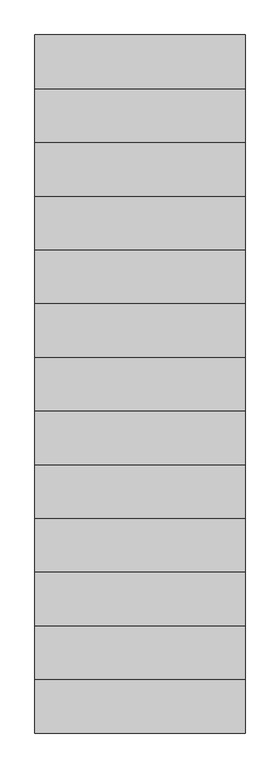
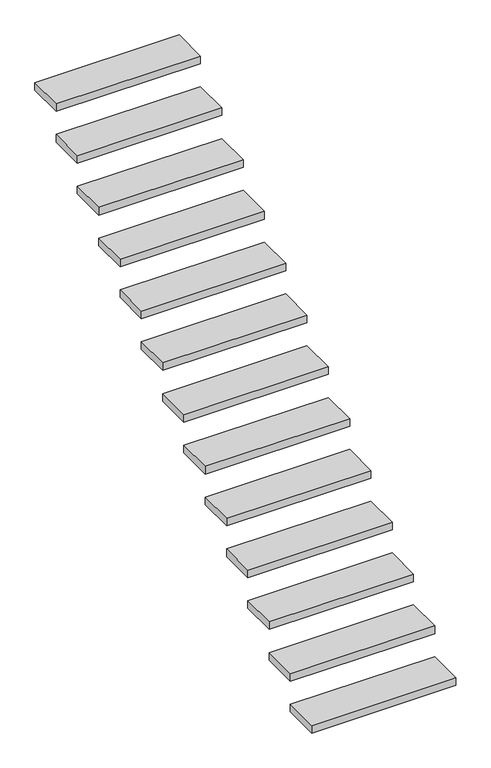
"""IFC4 building model written with IfcOpenShell, lengths in millimetres: stair geometry,   150832 :   150832."""

import ifcopenshell
import ifcopenshell.guid

model = None  # the IFC model being written
_history = None  # IfcOwnerHistory: only IFC2X3 demands one
_inside = {}  # id of a spatial element -> (the spatial element, [elements in it])
_under = {}  # id of a project, library or spatial element -> (it, [spatial elements below it])
_declared = {}  # id of a project -> (the project, [libraries it declares])
_typed = {}  # id of a type object -> (the type object, [elements of that type])
_made_of = {}  # id of a material, layer set ... -> (it, [elements and type objects made of it])


def new_model(schema):
    """Start an empty IFC model of exactly this schema.

    Asked for "IFC4X3", IfcOpenShell would pick the latest addendum, in which some entities
    have other attributes; the version numbers below select the first issue.
    IFC2X3 requires an IfcOwnerHistory on every rooted entity: one is made here for all.
    """
    global model, _history
    if schema == "IFC4X3":
        model = ifcopenshell.file(schema_version=(4, 3, 0, 0))
    else:
        model = ifcopenshell.file(schema=schema)
    _inside.clear()
    _under.clear()
    _declared.clear()
    _typed.clear()
    _made_of.clear()
    _history = None
    if model.schema == "IFC2X3":
        org = make("IfcOrganization", Name="unknown")
        user = make(
            "IfcPersonAndOrganization",
            ThePerson=make("IfcPerson", FamilyName="unknown"),
            TheOrganization=org,
        )
        app = make(
            "IfcApplication",
            ApplicationDeveloper=org,
            Version="unknown",
            ApplicationFullName="unknown",
            ApplicationIdentifier="unknown",
        )
        _history = make(
            "IfcOwnerHistory",
            OwningUser=user,
            OwningApplication=app,
            ChangeAction="ADDED",
            CreationDate=0,
        )
    return model


def make(cls, **values):
    """One entity of the class cls with the attributes given. An attribute that is None is left unset."""
    return model.create_entity(
        cls, **{name: value for name, value in values.items() if value is not None}
    )


def rooted(cls, **values):
    """An entity with a GlobalId (a new one), such as an element, a storey or a relation."""
    return make(cls, GlobalId=ifcopenshell.guid.new(), OwnerHistory=_history, **values)


def si_unit(unit_type, name, prefix=None):
    """IfcSIUnit, for example si_unit("LENGTHUNIT", "METRE", prefix="MILLI")."""
    return make("IfcSIUnit", UnitType=unit_type, Prefix=prefix, Name=name)


def assignment(units):
    """IfcUnitAssignment: the units of a project."""
    return None if units is None else make("IfcUnitAssignment", Units=units)


def point(xyz):
    """IfcCartesianPoint."""
    return None if xyz is None else make("IfcCartesianPoint", Coordinates=xyz)


def direction(xyz):
    """IfcDirection."""
    return None if xyz is None else make("IfcDirection", DirectionRatios=xyz)


def frame(location, z_axis=None, x_axis=None):
    """IfcAxis2Placement3D, a coordinate frame: its origin and axes. An axis left out is left unset."""
    return make(
        "IfcAxis2Placement3D",
        Location=point(location),
        Axis=direction(z_axis),
        RefDirection=direction(x_axis),
    )


def origin():
    """The frame at (0, 0, 0) with its axes left unset."""
    return frame((0.0, 0.0, 0.0))


def place(relative_to, where):
    """IfcLocalPlacement: puts the frame where relative to a parent placement (None: the world)."""
    return make(
        "IfcLocalPlacement", PlacementRelTo=relative_to, RelativePlacement=where
    )


def context(
    kind, dimensions, precision=None, world=None, true_north=None, identifier=None
):
    """IfcGeometricRepresentationContext, for example the 3D "Model" context."""
    return make(
        "IfcGeometricRepresentationContext",
        ContextIdentifier=identifier,
        ContextType=kind,
        CoordinateSpaceDimension=dimensions,
        Precision=precision,
        WorldCoordinateSystem=world,
        TrueNorth=true_north,
    )


def project(units=None, contexts=None):
    """IfcProject with its units and contexts."""
    return rooted(
        "IfcProject",
        Name="project",
        RepresentationContexts=contexts,
        UnitsInContext=assignment(units),
    )


def spatial(cls, under=None, at=None, **own):
    """A site, building, storey or space (cls), placed at a placement, below another one or the project."""
    s = rooted(cls, ObjectPlacement=at, **own)
    if under is not None:
        _under.setdefault(under.id(), (under, []))[1].append(s)
    return s


def polyline(points):
    """IfcPolyline through the points."""
    return make("IfcPolyline", Points=[point(p) for p in points])


def outline(outer, holes=None, kind="AREA"):
    """IfcArbitraryClosedProfileDef: a profile drawn as a closed curve; with holes, ...WithVoids."""
    if holes is None:
        return make("IfcArbitraryClosedProfileDef", ProfileType=kind, OuterCurve=outer)
    return make(
        "IfcArbitraryProfileDefWithVoids",
        ProfileType=kind,
        OuterCurve=outer,
        InnerCurves=holes,
    )


def extrude(swept, where, along, depth):
    """IfcExtrudedAreaSolid: the profile swept, set in the frame where, extruded along a direction by depth."""
    return make(
        "IfcExtrudedAreaSolid",
        SweptArea=swept,
        Position=where,
        ExtrudedDirection=direction(along),
        Depth=depth,
    )


def shape(context_of_items, identifier, shape_type, items):
    """IfcShapeRepresentation: the items that make up one representation, for example the "Body"."""
    return make(
        "IfcShapeRepresentation",
        ContextOfItems=context_of_items,
        RepresentationIdentifier=identifier,
        RepresentationType=shape_type,
        Items=items,
    )


def source(mapping_origin, context_of_items, identifier, shape_type, items):
    """IfcRepresentationMap: a shape defined once, which mapped items show again and again."""
    return make(
        "IfcRepresentationMap",
        MappingOrigin=mapping_origin,
        MappedRepresentation=shape(context_of_items, identifier, shape_type, items),
    )


def transform(
    local_origin,
    x_axis=None,
    y_axis=None,
    z_axis=None,
    scale=None,
    scale2=None,
    scale3=None,
    uniform=True,
):
    """IfcCartesianTransformationOperator3D, or its non-uniform kind. x_axis, y_axis, z_axis: its Axis1, 2, 3."""
    if uniform:
        return make(
            "IfcCartesianTransformationOperator3D",
            Axis1=direction(x_axis),
            Axis2=direction(y_axis),
            LocalOrigin=point(local_origin),
            Scale=scale,
            Axis3=direction(z_axis),
        )
    return make(
        "IfcCartesianTransformationOperator3DnonUniform",
        Axis1=direction(x_axis),
        Axis2=direction(y_axis),
        LocalOrigin=point(local_origin),
        Scale=scale,
        Axis3=direction(z_axis),
        Scale2=scale2,
        Scale3=scale3,
    )


def mapped(mapping_source, mapping_target):
    """IfcMappedItem: shows the shape of a source again, moved by a transform."""
    return make(
        "IfcMappedItem", MappingSource=mapping_source, MappingTarget=mapping_target
    )


def made_of(thing, what):
    """Note that an element or type object is made of a material, layer set ...; save() writes the relation."""
    if what is not None:
        _made_of.setdefault(what.id(), (what, []))[1].append(thing)
    return thing


def element(
    cls,
    number,
    at=None,
    inside=None,
    cuts=None,
    type_object=None,
    material=None,
    context=None,
    identifier="Body",
    shape_type=None,
    held_by="IfcProductDefinitionShape",
    body=None,
    shapes=None,
    **own,
):
    """One element of the class cls, such as IfcWall. Its Tag is "e" and its number.

    at: its placement. inside: the storey or other place that contains it. cuts: it is an
    opening in that element (IfcRelVoidsElement). A single representation is given by context,
    identifier, shape_type and body (its items); several are given by shapes. held_by: the class
    of the entity that holds the representations. save() writes the other relations.
    """
    e = rooted(cls, Tag="e%d" % number, ObjectPlacement=at, **own)
    if body is not None:
        shapes = [shape(context, identifier, shape_type, body)]
    if shapes is not None:
        e.Representation = make(held_by, Representations=shapes)
    if inside is not None:
        _inside.setdefault(inside.id(), (inside, []))[1].append(e)
    if cuts is not None:
        rooted(
            "IfcRelVoidsElement", RelatingBuildingElement=cuts, RelatedOpeningElement=e
        )
    if type_object is not None:
        _typed.setdefault(type_object.id(), (type_object, []))[1].append(e)
    return made_of(e, material)


def aggregate(whole, parts):
    """IfcRelAggregates: a whole, such as a stair, and the parts it consists of."""
    return rooted("IfcRelAggregates", RelatingObject=whole, RelatedObjects=parts)


def save(model, path):
    """Write the relations noted so far, then the file.

    IfcRelAggregates (storeys below a building ...), IfcRelContainedInSpatialStructure (elements
    in a storey), IfcRelDefinesByType, IfcRelAssociatesMaterial and IfcRelDeclares: one each for
    every whole, place, type object, material and project.
    """
    for whole, parts in _under.values():
        aggregate(whole, parts)
    for where, things in _inside.values():
        rooted(
            "IfcRelContainedInSpatialStructure",
            RelatedElements=things,
            RelatingStructure=where,
        )
    for kind, things in _typed.values():
        rooted("IfcRelDefinesByType", RelatedObjects=things, RelatingType=kind)
    for what, things in _made_of.values():
        rooted("IfcRelAssociatesMaterial", RelatedObjects=things, RelatingMaterial=what)
    for by, libraries in _declared.values():
        rooted("IfcRelDeclares", RelatingContext=by, RelatedDefinitions=libraries)
    model.write(path)


def stair_42ef58a3(model_context):
    return source(origin(), model_context, "Body", "SweptSolid", [
        extrude(outline(polyline([(165697.7593015, 42144.7962965), (165697.7593015, 41914.7962965), (164797.7593015, 41914.7962965), (164797.7593015, 42144.7962965), (165697.7593015, 42144.7962965)])), frame((0.0, 0.0, 3482.1428571), z_axis=(0.0, 0.0, 1.0), x_axis=(1.0, 0.0, 0.0)), (0.0, 0.0, 1.0), 50.0),
        extrude(outline(polyline([(165697.7593015, 42374.7962965), (165697.7593015, 42144.7962965), (164797.7593015, 42144.7962965), (164797.7593015, 42374.7962965), (165697.7593015, 42374.7962965)])), frame((0.0, 0.0, 3684.2857143), z_axis=(0.0, 0.0, 1.0), x_axis=(1.0, 0.0, 0.0)), (0.0, 0.0, 1.0), 50.0),
        extrude(outline(polyline([(165697.7593015, 42604.7962965), (165697.7593015, 42374.7962965), (164797.7593015, 42374.7962965), (164797.7593015, 42604.7962965), (165697.7593015, 42604.7962965)])), frame((0.0, 0.0, 3886.4285714), z_axis=(0.0, 0.0, 1.0), x_axis=(1.0, 0.0, 0.0)), (0.0, 0.0, 1.0), 50.0),
        extrude(outline(polyline([(165697.7593015, 42834.7962965), (165697.7593015, 42604.7962965), (164797.7593015, 42604.7962965), (164797.7593015, 42834.7962965), (165697.7593015, 42834.7962965)])), frame((0.0, 0.0, 4088.5714286), z_axis=(0.0, 0.0, 1.0), x_axis=(1.0, 0.0, 0.0)), (0.0, 0.0, 1.0), 50.0),
        extrude(outline(polyline([(165697.7593015, 43064.7962965), (165697.7593015, 42834.7962965), (164797.7593015, 42834.7962965), (164797.7593015, 43064.7962965), (165697.7593015, 43064.7962965)])), frame((0.0, 0.0, 4290.7142857), z_axis=(0.0, 0.0, 1.0), x_axis=(1.0, 0.0, 0.0)), (0.0, 0.0, 1.0), 50.0),
        extrude(outline(polyline([(165697.7593015, 43294.7962965), (165697.7593015, 43064.7962965), (164797.7593015, 43064.7962965), (164797.7593015, 43294.7962965), (165697.7593015, 43294.7962965)])), frame((0.0, 0.0, 4492.8571429), z_axis=(0.0, 0.0, 1.0), x_axis=(1.0, 0.0, 0.0)), (0.0, 0.0, 1.0), 50.0),
        extrude(outline(polyline([(165697.7593015, 43524.7962965), (165697.7593015, 43294.7962965), (164797.7593015, 43294.7962965), (164797.7593015, 43524.7962965), (165697.7593015, 43524.7962965)])), frame((0.0, 0.0, 4695.0), z_axis=(0.0, 0.0, 1.0), x_axis=(1.0, 0.0, 0.0)), (0.0, 0.0, 1.0), 50.0),
        extrude(outline(polyline([(165697.7593015, 43754.7962965), (165697.7593015, 43524.7962965), (164797.7593015, 43524.7962965), (164797.7593015, 43754.7962965), (165697.7593015, 43754.7962965)])), frame((0.0, 0.0, 4897.1428571), z_axis=(0.0, 0.0, 1.0), x_axis=(1.0, 0.0, 0.0)), (0.0, 0.0, 1.0), 50.0),
        extrude(outline(polyline([(165697.7593015, 43984.7962965), (165697.7593015, 43754.7962965), (164797.7593015, 43754.7962965), (164797.7593015, 43984.7962965), (165697.7593015, 43984.7962965)])), frame((0.0, 0.0, 5099.2857143), z_axis=(0.0, 0.0, 1.0), x_axis=(1.0, 0.0, 0.0)), (0.0, 0.0, 1.0), 50.0),
        extrude(outline(polyline([(165697.7593015, 44214.7962965), (165697.7593015, 43984.7962965), (164797.7593015, 43984.7962965), (164797.7593015, 44214.7962965), (165697.7593015, 44214.7962965)])), frame((0.0, 0.0, 5301.4285714), z_axis=(0.0, 0.0, 1.0), x_axis=(1.0, 0.0, 0.0)), (0.0, 0.0, 1.0), 50.0),
        extrude(outline(polyline([(165697.7593015, 44444.7962965), (165697.7593015, 44214.7962965), (164797.7593015, 44214.7962965), (164797.7593015, 44444.7962965), (165697.7593015, 44444.7962965)])), frame((0.0, 0.0, 5503.5714286), z_axis=(0.0, 0.0, 1.0), x_axis=(1.0, 0.0, 0.0)), (0.0, 0.0, 1.0), 50.0),
        extrude(outline(polyline([(165697.7593015, 44674.7962965), (165697.7593015, 44444.7962965), (164797.7593015, 44444.7962965), (164797.7593015, 44674.7962965), (165697.7593015, 44674.7962965)])), frame((0.0, 0.0, 5705.7142857), z_axis=(0.0, 0.0, 1.0), x_axis=(1.0, 0.0, 0.0)), (0.0, 0.0, 1.0), 50.0),
        extrude(outline(polyline([(165697.7593015, 44904.7962965), (165697.7593015, 44674.7962965), (164797.7593015, 44674.7962965), (164797.7593015, 44904.7962965), (165697.7593015, 44904.7962965)])), frame((0.0, 0.0, 5907.8571429), z_axis=(0.0, 0.0, 1.0), x_axis=(1.0, 0.0, 0.0)), (0.0, 0.0, 1.0), 50.0),
    ])


if __name__ == "__main__":
    model = new_model("IFC4")
    model_context = context("Model", 3, world=origin())
    ifc_project = project(units=[si_unit("LENGTHUNIT", "METRE", prefix="MILLI")], contexts=[model_context])
    site = spatial("IfcSite", under=ifc_project)
    building = spatial("IfcBuilding", under=site)
    placement = place(None, origin())
    stair_shape = stair_42ef58a3(model_context)
    element("IfcStair", 1, ObjectType="  150832 :   150832", at=placement, inside=building, context=model_context, shape_type="MappedRepresentation", body=[
        mapped(stair_shape, transform((0.0, 0.0, 0.0), x_axis=(1.0, 0.0, 0.0), y_axis=(0.0, 1.0, 0.0), z_axis=(0.0, 0.0, 1.0))),
    ])
    save(model, "model.ifc")

# Revit data of these elements
# Type "  150832 :   150832"
#   Abrechnungsart = "St"
#   Allright_Bauteil_ID = "0131Tre0659044593"
#   Codetext = "TR-MASSIV-GER\\"
#   Material = "Stahlbeton"
#   Objektname = "Treppe"
#   NameOverride = " "
#   Reference = "STB-Treppe"
#   ThermalTransmittance = 0.0000 BTU/(h·ft²·°F)
#   NosingLength = 0.000 m
#   NumberOfRiser = 14
#   NumberOfTreads = 13
#   RiserHeight = 2.021 m
#   TreadLength = 2.300 m
#   IsExternal = no
#   FireExit = no
#   HandicapAccessible = no
#   HasNonSkidSurface = no
# Element 1 (IfcStair, "  150832 :   150832")
#   Materials on its faces: "weiss"
# Materials
#   "weiss": class "Unassigned", colour RGB 255 255 255, transparency 0
